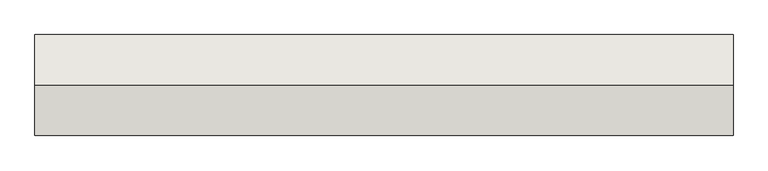
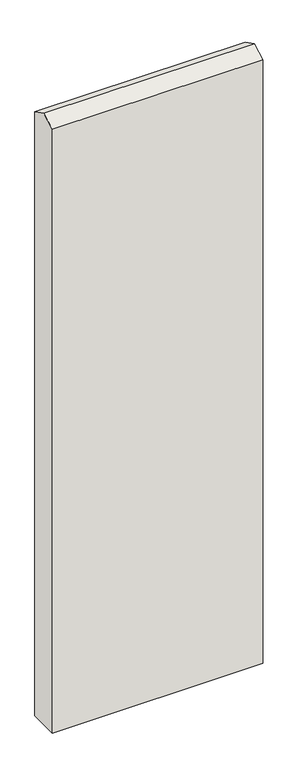
"""IFC4 building model written with IfcOpenShell, lengths in millimetres: wall geometry, Holzwand."""

from ifc_helpers import new_model, si_unit, frame, origin, place, context, project, spatial, polyline, outline, extrude, source, transform, mapped, element, save


def wall_95dfda24(model_context):
    return source(origin(), model_context, "Body", "SweptSolid", [
        extrude(outline(polyline([(100.0, 4251.6781465), (200.0, 4200.7256015), (200.0, 0.0), (0.0, 0.0), (0.0, 4200.7256015), (100.0, 4251.6781465)])), frame((0.0, 0.0, 0.0), z_axis=(1.0, 0.0, 0.0), x_axis=(0.0, 1.0, 0.0)), (0.0, 0.0, 1.0), 1385.0),
    ])


if __name__ == "__main__":
    model = new_model("IFC4")
    model_context = context("Model", 3, world=origin())
    ifc_project = project(units=[si_unit("LENGTHUNIT", "METRE", prefix="MILLI")], contexts=[model_context])
    site = spatial("IfcSite", under=ifc_project)
    building = spatial("IfcBuilding", under=site)
    placement = place(None, origin())
    wall_shape = wall_95dfda24(model_context)
    element("IfcWall", 1, ObjectType="Holzwand", at=placement, inside=building, context=model_context, shape_type="MappedRepresentation", body=[
        mapped(wall_shape, transform((0.0, 0.0, 0.0), x_axis=(1.0, 0.0, 0.0), y_axis=(0.0, 1.0, 0.0), z_axis=(0.0, 0.0, 1.0))),
    ])
    save(model, "model.ifc")

# Revit data of these elements
# Element 1 (IfcWall, "Holzwand")
#   Materials on its faces: "holzschalung"
# Materials
#   "holzschalung": class "Unassigned", colour RGB 128 128 128, transparency 0
